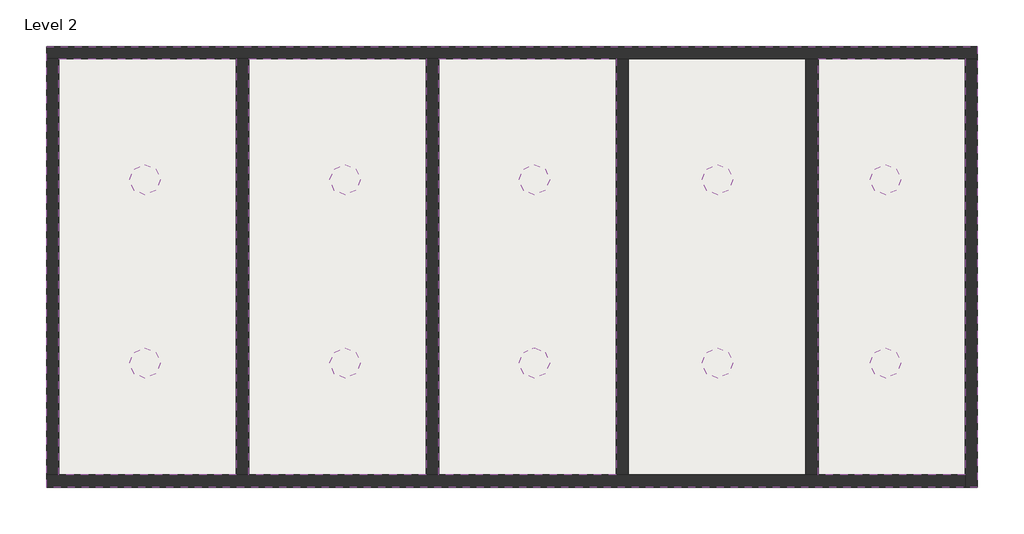
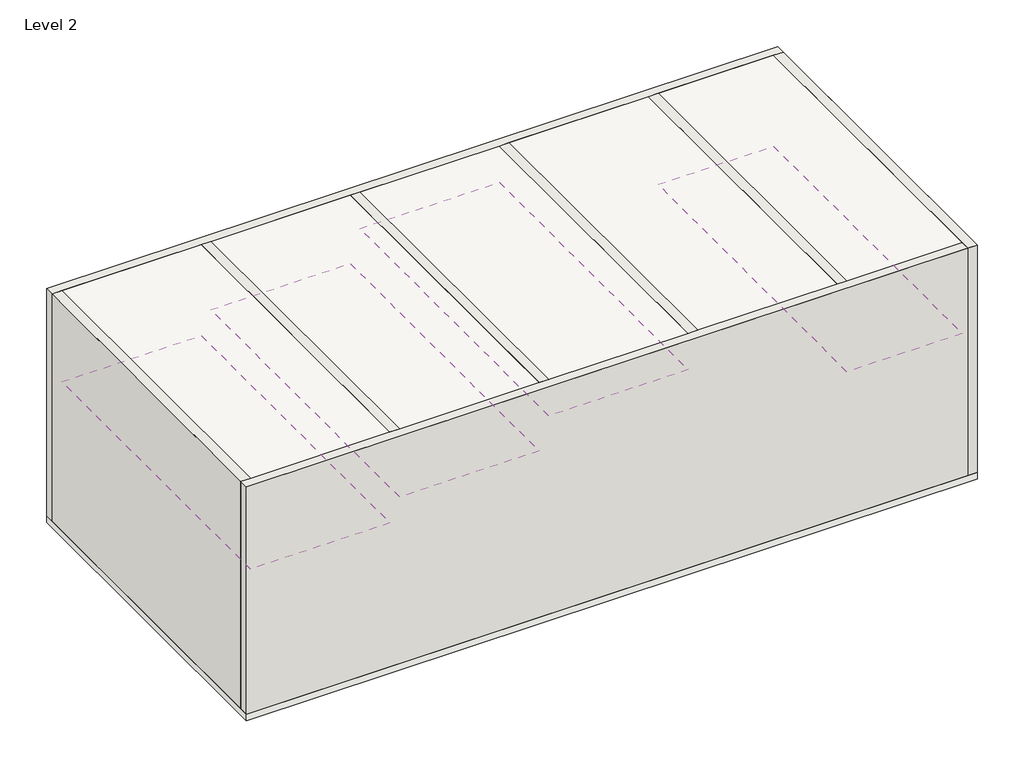
# One storey: 10 light fixtures, 8 walls, 4 coverings, 2 slabs.
"""IFC4 building model written with IfcOpenShell, lengths in millimetres."""

import ifcopenshell
import ifcopenshell.guid

model = None  # the IFC model being written
_history = None  # IfcOwnerHistory: only IFC2X3 demands one
_inside = {}  # id of a spatial element -> (the spatial element, [elements in it])
_under = {}  # id of a project, library or spatial element -> (it, [spatial elements below it])
_declared = {}  # id of a project -> (the project, [libraries it declares])
_typed = {}  # id of a type object -> (the type object, [elements of that type])
_made_of = {}  # id of a material, layer set ... -> (it, [elements and type objects made of it])


def new_model(schema):
    """Start an empty IFC model of exactly this schema.

    Asked for "IFC4X3", IfcOpenShell would pick the latest addendum, in which some entities
    have other attributes; the version numbers below select the first issue.
    IFC2X3 requires an IfcOwnerHistory on every rooted entity: one is made here for all.
    """
    global model, _history
    if schema == "IFC4X3":
        model = ifcopenshell.file(schema_version=(4, 3, 0, 0))
    else:
        model = ifcopenshell.file(schema=schema)
    _inside.clear()
    _under.clear()
    _declared.clear()
    _typed.clear()
    _made_of.clear()
    _history = None
    if model.schema == "IFC2X3":
        org = make("IfcOrganization", Name="unknown")
        user = make(
            "IfcPersonAndOrganization",
            ThePerson=make("IfcPerson", FamilyName="unknown"),
            TheOrganization=org,
        )
        app = make(
            "IfcApplication",
            ApplicationDeveloper=org,
            Version="unknown",
            ApplicationFullName="unknown",
            ApplicationIdentifier="unknown",
        )
        _history = make(
            "IfcOwnerHistory",
            OwningUser=user,
            OwningApplication=app,
            ChangeAction="ADDED",
            CreationDate=0,
        )
    return model


def make(cls, **values):
    """One entity of the class cls with the attributes given. An attribute that is None is left unset."""
    return model.create_entity(
        cls, **{name: value for name, value in values.items() if value is not None}
    )


def rooted(cls, **values):
    """An entity with a GlobalId (a new one), such as an element, a storey or a relation."""
    return make(cls, GlobalId=ifcopenshell.guid.new(), OwnerHistory=_history, **values)


def si_unit(unit_type, name, prefix=None):
    """IfcSIUnit, for example si_unit("LENGTHUNIT", "METRE", prefix="MILLI")."""
    return make("IfcSIUnit", UnitType=unit_type, Prefix=prefix, Name=name)


def assignment(units):
    """IfcUnitAssignment: the units of a project."""
    return None if units is None else make("IfcUnitAssignment", Units=units)


def point(xyz):
    """IfcCartesianPoint."""
    return None if xyz is None else make("IfcCartesianPoint", Coordinates=xyz)


def direction(xyz):
    """IfcDirection."""
    return None if xyz is None else make("IfcDirection", DirectionRatios=xyz)


def frame(location, z_axis=None, x_axis=None):
    """IfcAxis2Placement3D, a coordinate frame: its origin and axes. An axis left out is left unset."""
    return make(
        "IfcAxis2Placement3D",
        Location=point(location),
        Axis=direction(z_axis),
        RefDirection=direction(x_axis),
    )


def frame_2d(location, x_axis=None):
    """IfcAxis2Placement2D, a coordinate frame in the plane: its origin and x axis."""
    return make(
        "IfcAxis2Placement2D", Location=point(location), RefDirection=direction(x_axis)
    )


def origin():
    """The frame at (0, 0, 0) with its axes left unset."""
    return frame((0.0, 0.0, 0.0))


def origin_2d():
    """The frame at (0, 0) in the plane with its x axis left unset."""
    return frame_2d((0.0, 0.0))


def place(relative_to, where):
    """IfcLocalPlacement: puts the frame where relative to a parent placement (None: the world)."""
    return make(
        "IfcLocalPlacement", PlacementRelTo=relative_to, RelativePlacement=where
    )


def context(
    kind, dimensions, precision=None, world=None, true_north=None, identifier=None
):
    """IfcGeometricRepresentationContext, for example the 3D "Model" context."""
    return make(
        "IfcGeometricRepresentationContext",
        ContextIdentifier=identifier,
        ContextType=kind,
        CoordinateSpaceDimension=dimensions,
        Precision=precision,
        WorldCoordinateSystem=world,
        TrueNorth=true_north,
    )


def project(units=None, contexts=None):
    """IfcProject with its units and contexts."""
    return rooted(
        "IfcProject",
        Name="project",
        RepresentationContexts=contexts,
        UnitsInContext=assignment(units),
    )


def spatial(cls, under=None, at=None, **own):
    """A site, building, storey or space (cls), placed at a placement, below another one or the project."""
    s = rooted(cls, ObjectPlacement=at, **own)
    if under is not None:
        _under.setdefault(under.id(), (under, []))[1].append(s)
    return s


def polyline(points):
    """IfcPolyline through the points."""
    return make("IfcPolyline", Points=[point(p) for p in points])


def circle_curve(where, radius):
    """IfcCircle in the frame where."""
    return make("IfcCircle", Position=where, Radius=radius)


def ellipse_curve(where, semi_axis1, semi_axis2):
    """IfcEllipse in the frame where."""
    return make(
        "IfcEllipse", Position=where, SemiAxis1=semi_axis1, SemiAxis2=semi_axis2
    )


def trimmed(basis, trim1, trim2, sense, master):
    """IfcTrimmedCurve: the piece of a basis curve between two trims."""
    return make(
        "IfcTrimmedCurve",
        BasisCurve=basis,
        Trim1=trim1,
        Trim2=trim2,
        SenseAgreement=sense,
        MasterRepresentation=master,
    )


def segment(curve, same_sense, transition):
    """IfcCompositeCurveSegment."""
    return make(
        "IfcCompositeCurveSegment",
        Transition=transition,
        SameSense=same_sense,
        ParentCurve=curve,
    )


def composite_curve(segments, self_intersect=None):
    """IfcCompositeCurve: segments joined end to end."""
    return make("IfcCompositeCurve", Segments=segments, SelfIntersect=self_intersect)


def outline(outer, holes=None, kind="AREA"):
    """IfcArbitraryClosedProfileDef: a profile drawn as a closed curve; with holes, ...WithVoids."""
    if holes is None:
        return make("IfcArbitraryClosedProfileDef", ProfileType=kind, OuterCurve=outer)
    return make(
        "IfcArbitraryProfileDefWithVoids",
        ProfileType=kind,
        OuterCurve=outer,
        InnerCurves=holes,
    )


def extrude(swept, where, along, depth):
    """IfcExtrudedAreaSolid: the profile swept, set in the frame where, extruded along a direction by depth."""
    return make(
        "IfcExtrudedAreaSolid",
        SweptArea=swept,
        Position=where,
        ExtrudedDirection=direction(along),
        Depth=depth,
    )


def faces_of(points, faces, orient=None, outer=None):
    """IfcFace entities. A face is a list of loops; a loop is a list of indices into points, from 0.

    orient and outer hold one flag for each loop. By default every Orientation is true, the
    first loop of a face is its IfcFaceOuterBound and the others are IfcFaceBound.
    """
    made = []
    for i, loops in enumerate(faces):
        bounds = []
        for j, loop in enumerate(loops):
            is_outer = j == 0 if outer is None else outer[i][j]
            bounds.append(
                make(
                    "IfcFaceOuterBound" if is_outer else "IfcFaceBound",
                    Bound=make("IfcPolyLoop", Polygon=[points[k] for k in loop]),
                    Orientation=True if orient is None else orient[i][j],
                )
            )
        made.append(make("IfcFace", Bounds=bounds))
    return made


def faceted_brep(points, faces, orient=None, outer=None, voids=None):
    """IfcFacetedBrep: a solid bounded by flat faces; with voids (closed shells), ...WithVoids."""
    shared = [point(p) for p in points]
    hull = make("IfcClosedShell", CfsFaces=faces_of(shared, faces, orient, outer))
    if voids is None:
        return make("IfcFacetedBrep", Outer=hull)
    return make(
        "IfcFacetedBrepWithVoids",
        Outer=hull,
        Voids=[
            make(cls, CfsFaces=faces_of(shared, fs, o, b)) for cls, fs, o, b in voids
        ],
    )


def shape(context_of_items, identifier, shape_type, items):
    """IfcShapeRepresentation: the items that make up one representation, for example the "Body"."""
    return make(
        "IfcShapeRepresentation",
        ContextOfItems=context_of_items,
        RepresentationIdentifier=identifier,
        RepresentationType=shape_type,
        Items=items,
    )


def source(mapping_origin, context_of_items, identifier, shape_type, items):
    """IfcRepresentationMap: a shape defined once, which mapped items show again and again."""
    return make(
        "IfcRepresentationMap",
        MappingOrigin=mapping_origin,
        MappedRepresentation=shape(context_of_items, identifier, shape_type, items),
    )


def transform(
    local_origin,
    x_axis=None,
    y_axis=None,
    z_axis=None,
    scale=None,
    scale2=None,
    scale3=None,
    uniform=True,
):
    """IfcCartesianTransformationOperator3D, or its non-uniform kind. x_axis, y_axis, z_axis: its Axis1, 2, 3."""
    if uniform:
        return make(
            "IfcCartesianTransformationOperator3D",
            Axis1=direction(x_axis),
            Axis2=direction(y_axis),
            LocalOrigin=point(local_origin),
            Scale=scale,
            Axis3=direction(z_axis),
        )
    return make(
        "IfcCartesianTransformationOperator3DnonUniform",
        Axis1=direction(x_axis),
        Axis2=direction(y_axis),
        LocalOrigin=point(local_origin),
        Scale=scale,
        Axis3=direction(z_axis),
        Scale2=scale2,
        Scale3=scale3,
    )


def mapped(mapping_source, mapping_target):
    """IfcMappedItem: shows the shape of a source again, moved by a transform."""
    return make(
        "IfcMappedItem", MappingSource=mapping_source, MappingTarget=mapping_target
    )


def made_of(thing, what):
    """Note that an element or type object is made of a material, layer set ...; save() writes the relation."""
    if what is not None:
        _made_of.setdefault(what.id(), (what, []))[1].append(thing)
    return thing


def element(
    cls,
    number,
    at=None,
    inside=None,
    cuts=None,
    type_object=None,
    material=None,
    context=None,
    identifier="Body",
    shape_type=None,
    held_by="IfcProductDefinitionShape",
    body=None,
    shapes=None,
    **own,
):
    """One element of the class cls, such as IfcWall. Its Tag is "e" and its number.

    at: its placement. inside: the storey or other place that contains it. cuts: it is an
    opening in that element (IfcRelVoidsElement). A single representation is given by context,
    identifier, shape_type and body (its items); several are given by shapes. held_by: the class
    of the entity that holds the representations. save() writes the other relations.
    """
    e = rooted(cls, Tag="e%d" % number, ObjectPlacement=at, **own)
    if body is not None:
        shapes = [shape(context, identifier, shape_type, body)]
    if shapes is not None:
        e.Representation = make(held_by, Representations=shapes)
    if inside is not None:
        _inside.setdefault(inside.id(), (inside, []))[1].append(e)
    if cuts is not None:
        rooted(
            "IfcRelVoidsElement", RelatingBuildingElement=cuts, RelatedOpeningElement=e
        )
    if type_object is not None:
        _typed.setdefault(type_object.id(), (type_object, []))[1].append(e)
    return made_of(e, material)


def aggregate(whole, parts):
    """IfcRelAggregates: a whole, such as a stair, and the parts it consists of."""
    return rooted("IfcRelAggregates", RelatingObject=whole, RelatedObjects=parts)


def save(model, path):
    """Write the relations noted so far, then the file.

    IfcRelAggregates (storeys below a building ...), IfcRelContainedInSpatialStructure (elements
    in a storey), IfcRelDefinesByType, IfcRelAssociatesMaterial and IfcRelDeclares: one each for
    every whole, place, type object, material and project.
    """
    for whole, parts in _under.values():
        aggregate(whole, parts)
    for where, things in _inside.values():
        rooted(
            "IfcRelContainedInSpatialStructure",
            RelatedElements=things,
            RelatingStructure=where,
        )
    for kind, things in _typed.values():
        rooted("IfcRelDefinesByType", RelatedObjects=things, RelatingType=kind)
    for what, things in _made_of.values():
        rooted("IfcRelAssociatesMaterial", RelatedObjects=things, RelatingMaterial=what)
    for by, libraries in _declared.values():
        rooted("IfcRelDeclares", RelatingContext=by, RelatedDefinitions=libraries)
    model.write(path)


def plane_surface(at):
    """IfcPlane: the flat surface through the origin of the frame at, square to its z axis."""
    return make("IfcPlane", Position=at)


def revolved_surface(curve, axis_point, axis_direction):
    """IfcSurfaceOfRevolution: the curve turned about the line through axis_point along axis_direction."""
    return make(
        "IfcSurfaceOfRevolution",
        SweptCurve=make("IfcArbitraryOpenProfileDef", ProfileType="CURVE", Curve=curve),
        AxisPosition=make("IfcAxis1Placement", Location=point(axis_point), Axis=direction(axis_direction)),
    )


def advanced_brep(points, edges, surfaces, faces):
    """IfcAdvancedBrep: a solid bounded by faces that lie on surfaces and meet in shared edges.

    An edge is (start, end): straight between two places in points (the first is 0);
    or (start, end, curve); or (start, end, curve, False) where it runs against its curve.
    A face is (place in surfaces, loops), or (place, loops, False) where it looks against
    its surface's normal. A loop lists edges by number (the first is 1), with a minus sign
    where the edge is run from its end to its start. The first loop is the outer one.
    """
    corners = [point(p) for p in points]
    vertices = [make("IfcVertexPoint", VertexGeometry=c) for c in corners]
    made = []
    for start, end, *more in edges:
        made.append(
            make(
                "IfcEdgeCurve",
                EdgeStart=vertices[start],
                EdgeEnd=vertices[end],
                EdgeGeometry=more[0] if more else make("IfcPolyline", Points=[corners[start], corners[end]]),
                SameSense=more[1] if len(more) > 1 else True,
            )
        )
    hull = []
    for where, loops, *sense in faces:
        bounds = []
        for j, loop in enumerate(loops):
            ring = [make("IfcOrientedEdge", EdgeElement=made[abs(k) - 1], Orientation=k > 0) for k in loop]
            bounds.append(
                make(
                    "IfcFaceOuterBound" if j == 0 else "IfcFaceBound",
                    Bound=make("IfcEdgeLoop", EdgeList=ring),
                    Orientation=True,
                )
            )
        hull.append(make("IfcAdvancedFace", Bounds=bounds, FaceSurface=surfaces[where], SameSense=sense[0] if sense else True))
    return make("IfcAdvancedBrep", Outer=make("IfcClosedShell", CfsFaces=hull))


def downlight_downlight_e6a68a7d(model_context):
    return source(origin(), model_context, "Body", "SolidModel", [
        advanced_brep(
        [(-230.0, 0.0, 0.0), (230.0, 0.0, 0.0), (0.0, 0.0, 0.0), (0.0, 0.0, 70.3180567)],
        [
            (0, 1, circle_curve(frame((0.0, 0.0, 0.0), z_axis=(0.0, 0.0, -1.0), x_axis=(1.0, 0.0, 0.0)), 230.0)),
            (1, 2),
            (2, 0),
            (1, 0, circle_curve(frame((0.0, 0.0, 0.0), z_axis=(0.0, 0.0, -1.0), x_axis=(1.0, 0.0, 0.0)), 230.0)),
            (3, 1, circle_curve(frame((13.1969865, 0.0, -297.8236248), z_axis=(0.0, 1.0, 0.0), x_axis=(1.0, 0.0, 0.0)), 368.3781456)),
            (0, 3, circle_curve(frame((-13.1969865, 0.0, -297.8236248), z_axis=(0.0, 1.0, 0.0), x_axis=(-1.0, 0.0, 0.0)), 368.3781456)),
        ],
        [
            plane_surface(frame((0.0, 0.0, 0.0), z_axis=(0.0, 0.0, -1.0), x_axis=(1.0, 0.0, 0.0))),
            revolved_surface(trimmed(ellipse_curve(frame((13.1969865, 0.0, -297.8236248), z_axis=(0.0, -1.0, 0.0), x_axis=(1.0, 0.0, 0.0)), 368.3781456, 368.3781456), [point((230.0, 0.0, 0.0))], [point((0.0, 0.0, 70.3180567))], True, "CARTESIAN"), (0.0, 0.0, 2194.0651339), (0.0, 0.0, 1.0)),
        ],
        [
            (0, [[1, 2, 3]]),
            (0, [[4, -3, -2]]),
            (1, [[5, -1, 6]]),
            (1, [[-6, -4, -5]]),
        ],
    ),
        extrude(outline(composite_curve([segment(trimmed(circle_curve(origin_2d(), 250.0), [point((-250.0, 0.0))], [point((250.0, 0.0))], False, "CARTESIAN"), True, "CONTINUOUS"), segment(trimmed(circle_curve(origin_2d(), 250.0), [point((250.0, 0.0))], [point((-250.0, 0.0))], False, "CARTESIAN"), True, "CONTINUOUS")], self_intersect=False)), frame((0.0, 0.0, -10.1537533), z_axis=(0.0, 0.0, 1.0), x_axis=(1.0, 0.0, 0.0)), (0.0, 0.0, 1.0), 10.1537533),
    ])


model = new_model("IFC4")

# Units and contexts
model_context = context("Model", 3, world=origin())
ifc_project = project(units=[si_unit("LENGTHUNIT", "METRE", prefix="MILLI")], contexts=[model_context])

# Site, building, storey
site = spatial("IfcSite", under=ifc_project)
building = spatial("IfcBuilding", under=site)
storey = spatial("IfcBuildingStorey", under=building, Name="Level 2", Elevation=5000.0)

# Coverings
placement = place(None, origin())
element("IfcCovering", 1, ObjectType="Plain", at=placement, inside=storey, context=model_context, shape_type="SweptSolid", body=[
    extrude(outline(polyline([(4711.6370984, -2494.7382368), (4711.6370984, 4305.2617632), (7111.6370984, 4305.2617632), (7111.6370984, -2494.7382368), (4711.6370984, -2494.7382368)])), frame((0.0, 0.0, 8000.0), z_axis=(0.0, 0.0, 1.0), x_axis=(1.0, 0.0, 0.0)), (0.0, 0.0, 1.0), 57.0),
])
element("IfcCovering", 2, ObjectType="Plain", at=placement, inside=storey, context=model_context, shape_type="SweptSolid", body=[
    extrude(outline(polyline([(-1488.3629016, -2494.7382368), (-1488.3629016, 4305.2617632), (1411.6370984, 4305.2617632), (1411.6370984, -2494.7382368), (-1488.3629016, -2494.7382368)])), frame((0.0, 0.0, 9200.0), z_axis=(0.0, 0.0, 1.0), x_axis=(1.0, 0.0, 0.0)), (0.0, 0.0, 1.0), 57.0),
])
element("IfcCovering", 3, ObjectType="Plain", at=placement, inside=storey, context=model_context, shape_type="SweptSolid", body=[
    extrude(outline(polyline([(-4588.3629016, -2494.7382368), (-4588.3629016, 4305.2617632), (-1688.3629016, 4305.2617632), (-1688.3629016, -2494.7382368), (-4588.3629016, -2494.7382368)])), frame((0.0, 0.0, 8500.0), z_axis=(0.0, 0.0, 1.0), x_axis=(1.0, 0.0, 0.0)), (0.0, 0.0, 1.0), 57.0),
])
element("IfcCovering", 4, ObjectType="Plain", at=placement, inside=storey, context=model_context, shape_type="SweptSolid", body=[
    extrude(outline(polyline([(-7688.3629016, 4305.2617632), (-4788.3629016, 4305.2617632), (-4788.3629016, -2494.7382368), (-7688.3629016, -2494.7382368), (-7688.3629016, 4305.2617632)])), frame((0.0, 0.0, 8000.0), z_axis=(0.0, 0.0, 1.0), x_axis=(1.0, 0.0, 0.0)), (0.0, 0.0, 1.0), 57.0),
])

# Light fixtures
downlight_downlight_shape = downlight_downlight_e6a68a7d(model_context)
element("IfcLightFixture", 5, ObjectType="Downlight : Downlight", at=placement, inside=storey, context=model_context, shape_type="MappedRepresentation", body=[
    mapped(downlight_downlight_shape, transform((-6281.2033206, -666.9973068, 7700.0), x_axis=(1.0, 0.0, 0.0), y_axis=(0.0, 1.0, 0.0), z_axis=(0.0, 0.0, 1.0))),
])
element("IfcLightFixture", 6, ObjectType="Downlight : Downlight", at=placement, inside=storey, context=model_context, shape_type="MappedRepresentation", body=[
    mapped(downlight_downlight_shape, transform((-6281.2033206, 2328.2026932, 7700.0), x_axis=(1.0, 0.0, 0.0), y_axis=(0.0, 1.0, 0.0), z_axis=(0.0, 0.0, 1.0))),
])
element("IfcLightFixture", 7, ObjectType="Downlight : Downlight", at=placement, inside=storey, context=model_context, shape_type="MappedRepresentation", body=[
    mapped(downlight_downlight_shape, transform((-3013.7777439, -666.9973068, 8800.0), x_axis=(1.0, 0.0, 0.0), y_axis=(0.0, 1.0, 0.0), z_axis=(0.0, 0.0, 1.0))),
])
element("IfcLightFixture", 8, ObjectType="Downlight : Downlight", at=placement, inside=storey, context=model_context, shape_type="MappedRepresentation", body=[
    mapped(downlight_downlight_shape, transform((-3013.7777439, 2328.2026932, 8800.0), x_axis=(1.0, 0.0, 0.0), y_axis=(0.0, 1.0, 0.0), z_axis=(0.0, 0.0, 1.0))),
])
element("IfcLightFixture", 9, ObjectType="Downlight : Downlight", at=placement, inside=storey, context=model_context, shape_type="MappedRepresentation", body=[
    mapped(downlight_downlight_shape, transform((76.5388311, -666.9973068, 8500.0), x_axis=(1.0, 0.0, 0.0), y_axis=(0.0, 1.0, 0.0), z_axis=(0.0, 0.0, 1.0))),
])
element("IfcLightFixture", 10, ObjectType="Downlight : Downlight", at=placement, inside=storey, context=model_context, shape_type="MappedRepresentation", body=[
    mapped(downlight_downlight_shape, transform((76.5388311, 2328.2026932, 8500.0), x_axis=(1.0, 0.0, 0.0), y_axis=(0.0, 1.0, 0.0), z_axis=(0.0, 0.0, 1.0))),
])
element("IfcLightFixture", 11, ObjectType="Downlight : Downlight", at=placement, inside=storey, context=model_context, shape_type="MappedRepresentation", body=[
    mapped(downlight_downlight_shape, transform((3067.3545284, -666.9973068, 8900.0), x_axis=(1.0, 0.0, 0.0), y_axis=(0.0, 1.0, 0.0), z_axis=(0.0, 0.0, 1.0))),
])
element("IfcLightFixture", 12, ObjectType="Downlight : Downlight", at=placement, inside=storey, context=model_context, shape_type="MappedRepresentation", body=[
    mapped(downlight_downlight_shape, transform((3067.3545284, 2328.2026932, 8900.0), x_axis=(1.0, 0.0, 0.0), y_axis=(0.0, 1.0, 0.0), z_axis=(0.0, 0.0, 1.0))),
])
element("IfcLightFixture", 13, ObjectType="Downlight : Downlight", at=placement, inside=storey, context=model_context, shape_type="MappedRepresentation", body=[
    mapped(downlight_downlight_shape, transform((5810.7393139, -666.9973068, 8000.0), x_axis=(1.0, 0.0, 0.0), y_axis=(0.0, 1.0, 0.0), z_axis=(0.0, 0.0, 1.0))),
])
element("IfcLightFixture", 14, ObjectType="Downlight : Downlight", at=placement, inside=storey, context=model_context, shape_type="MappedRepresentation", body=[
    mapped(downlight_downlight_shape, transform((5810.7393139, 2328.2026932, 8000.0), x_axis=(1.0, 0.0, 0.0), y_axis=(0.0, 1.0, 0.0), z_axis=(0.0, 0.0, 1.0))),
])

# Slabs
element("IfcSlab", 15, ObjectType="Generic 150mm", at=placement, inside=storey, context=model_context, shape_type="SweptSolid", body=[
    extrude(outline(polyline([(7311.6370984, 4505.2617632), (7311.6370984, -2694.7382368), (-7888.3629016, -2694.7382368), (-7888.3629016, 4505.2617632), (7311.6370984, 4505.2617632)])), frame((0.0, 0.0, 4850.0), z_axis=(0.0, 0.0, 1.0), x_axis=(1.0, 0.0, 0.0)), (0.0, 0.0, 1.0), 150.0),
])
element("IfcSlab", 16, ObjectType="Generic 150mm", at=placement, inside=storey, context=model_context, shape_type="SweptSolid", body=[
    extrude(outline(polyline([(7311.6370984, 4505.2617632), (7311.6370984, -2694.7382368), (-7888.3629016, -2694.7382368), (-7888.3629016, 4505.2617632), (7311.6370984, 4505.2617632)])), frame((0.0, 0.0, 9850.0), z_axis=(0.0, 0.0, 1.0), x_axis=(1.0, 0.0, 0.0)), (0.0, 0.0, 1.0), 150.0),
])

# Walls
element("IfcWall", 17, ObjectType="Generic - 200mm", at=placement, inside=storey, context=model_context, shape_type="Brep", body=[
    faceted_brep([(-7888.3629016, 4305.2617632, 5000.0), (-7688.3629016, 4305.2617632, 5000.0), (-4788.3629016, 4305.2617632, 5000.0), (-4588.3629016, 4305.2617632, 5000.0), (-1688.3629016, 4305.2617632, 5000.0), (-1488.3629016, 4305.2617632, 5000.0), (1411.6370984, 4305.2617632, 5000.0), (1611.6370984, 4305.2617632, 5000.0), (4511.6370984, 4305.2617632, 5000.0), (4711.6370984, 4305.2617632, 5000.0), (7111.6370984, 4305.2617632, 5000.0), (7311.6370984, 4305.2617632, 5000.0), (7311.6370984, 4305.2617632, 10000.0), (7111.6370984, 4305.2617632, 10000.0), (4711.6370984, 4305.2617632, 10000.0), (4511.6370984, 4305.2617632, 10000.0), (1611.6370984, 4305.2617632, 10000.0), (1411.6370984, 4305.2617632, 10000.0), (-1488.3629016, 4305.2617632, 10000.0), (-1688.3629016, 4305.2617632, 10000.0), (-4588.3629016, 4305.2617632, 10000.0), (-4788.3629016, 4305.2617632, 10000.0), (-7688.3629016, 4305.2617632, 10000.0), (-7888.3629016, 4305.2617632, 10000.0), (-7888.3629016, 4505.2617632, 5000.0), (-7888.3629016, 4505.2617632, 10000.0), (7311.6370984, 4505.2617632, 10000.0), (7311.6370984, 4505.2617632, 5000.0)], [[[0, 1, 2, 3, 4, 5, 6, 7, 8, 9, 10, 11, 12, 13, 14, 15, 16, 17, 18, 19, 20, 21, 22, 23]], [[24, 25, 26, 27]], [[11, 10, 9, 8, 7, 6, 5, 4, 3, 2, 1, 0, 24, 27]], [[23, 22, 21, 20, 19, 18, 17, 16, 15, 14, 13, 12, 26, 25]], [[12, 11, 27, 26]], [[0, 23, 25, 24]]]),
])
element("IfcWall", 18, ObjectType="Generic - 200mm", at=placement, inside=storey, context=model_context, shape_type="Brep", body=[
    faceted_brep([(7111.6370984, 4305.2617632, 5000.0), (7111.6370984, -2494.7382368, 5000.0), (7111.6370984, -2694.7382368, 5000.0), (7111.6370984, -2694.7382368, 10000.0), (7111.6370984, -2494.7382368, 10000.0), (7111.6370984, 4305.2617632, 10000.0), (7311.6370984, 4305.2617632, 5000.0), (7311.6370984, 4305.2617632, 10000.0), (7311.6370984, -2694.7382368, 10000.0), (7311.6370984, -2694.7382368, 5000.0)], [[[0, 1, 2, 3, 4, 5]], [[6, 7, 8, 9]], [[2, 1, 0, 6, 9]], [[5, 4, 3, 8, 7]], [[0, 5, 7, 6]], [[3, 2, 9, 8]]]),
])
element("IfcWall", 19, ObjectType="Generic - 200mm", at=placement, inside=storey, context=model_context, shape_type="Brep", body=[
    faceted_brep([(7111.6370984, -2494.7382368, 5000.0), (4711.6370984, -2494.7382368, 5000.0), (4511.6370984, -2494.7382368, 5000.0), (1611.6370984, -2494.7382368, 5000.0), (1411.6370984, -2494.7382368, 5000.0), (-1488.3629016, -2494.7382368, 5000.0), (-1688.3629016, -2494.7382368, 5000.0), (-4588.3629016, -2494.7382368, 5000.0), (-4788.3629016, -2494.7382368, 5000.0), (-7688.3629016, -2494.7382368, 5000.0), (-7888.3629016, -2494.7382368, 5000.0), (-7888.3629016, -2494.7382368, 10000.0), (-7688.3629016, -2494.7382368, 10000.0), (-4788.3629016, -2494.7382368, 10000.0), (-4588.3629016, -2494.7382368, 10000.0), (-1688.3629016, -2494.7382368, 10000.0), (-1488.3629016, -2494.7382368, 10000.0), (1411.6370984, -2494.7382368, 10000.0), (1611.6370984, -2494.7382368, 10000.0), (4511.6370984, -2494.7382368, 10000.0), (4711.6370984, -2494.7382368, 10000.0), (7111.6370984, -2494.7382368, 10000.0), (7111.6370984, -2694.7382368, 5000.0), (7111.6370984, -2694.7382368, 10000.0), (-7888.3629016, -2694.7382368, 10000.0), (-7888.3629016, -2694.7382368, 5000.0)], [[[0, 1, 2, 3, 4, 5, 6, 7, 8, 9, 10, 11, 12, 13, 14, 15, 16, 17, 18, 19, 20, 21]], [[22, 23, 24, 25]], [[10, 9, 8, 7, 6, 5, 4, 3, 2, 1, 0, 22, 25]], [[21, 20, 19, 18, 17, 16, 15, 14, 13, 12, 11, 24, 23]], [[0, 21, 23, 22]], [[11, 10, 25, 24]]]),
])
element("IfcWall", 20, ObjectType="Generic - 200mm", at=placement, inside=storey, context=model_context, shape_type="SweptSolid", body=[
    extrude(outline(polyline([(-7688.3629016, 4305.2617632), (-7688.3629016, -2494.7382368), (-7888.3629016, -2494.7382368), (-7888.3629016, 4305.2617632), (-7688.3629016, 4305.2617632)])), frame((0.0, 0.0, 5000.0), z_axis=(0.0, 0.0, 1.0), x_axis=(1.0, 0.0, 0.0)), (0.0, 0.0, 1.0), 5000.0),
])
element("IfcWall", 21, ObjectType="Generic - 200mm", at=placement, inside=storey, context=model_context, shape_type="SweptSolid", body=[
    extrude(outline(polyline([(-4788.3629016, -2494.7382368), (-4788.3629016, 4305.2617632), (-4588.3629016, 4305.2617632), (-4588.3629016, -2494.7382368), (-4788.3629016, -2494.7382368)])), frame((0.0, 0.0, 5000.0), z_axis=(0.0, 0.0, 1.0), x_axis=(1.0, 0.0, 0.0)), (0.0, 0.0, 1.0), 5000.0),
])
element("IfcWall", 22, ObjectType="Generic - 200mm", at=placement, inside=storey, context=model_context, shape_type="SweptSolid", body=[
    extrude(outline(polyline([(-1688.3629016, -2494.7382368), (-1688.3629016, 4305.2617632), (-1488.3629016, 4305.2617632), (-1488.3629016, -2494.7382368), (-1688.3629016, -2494.7382368)])), frame((0.0, 0.0, 5000.0), z_axis=(0.0, 0.0, 1.0), x_axis=(1.0, 0.0, 0.0)), (0.0, 0.0, 1.0), 5000.0),
])
element("IfcWall", 23, ObjectType="Generic - 200mm", at=placement, inside=storey, context=model_context, shape_type="SweptSolid", body=[
    extrude(outline(polyline([(1411.6370984, -2494.7382368), (1411.6370984, 4305.2617632), (1611.6370984, 4305.2617632), (1611.6370984, -2494.7382368), (1411.6370984, -2494.7382368)])), frame((0.0, 0.0, 5000.0), z_axis=(0.0, 0.0, 1.0), x_axis=(1.0, 0.0, 0.0)), (0.0, 0.0, 1.0), 5000.0),
])
element("IfcWall", 24, ObjectType="Generic - 200mm", at=placement, inside=storey, context=model_context, shape_type="SweptSolid", body=[
    extrude(outline(polyline([(4511.6370984, -2494.7382368), (4511.6370984, 4305.2617632), (4711.6370984, 4305.2617632), (4711.6370984, -2494.7382368), (4511.6370984, -2494.7382368)])), frame((0.0, 0.0, 5000.0), z_axis=(0.0, 0.0, 1.0), x_axis=(1.0, 0.0, 0.0)), (0.0, 0.0, 1.0), 5000.0),
])

save(model, "model.ifc")

# Revit data of these elements
# Type "Plain"
#   built-in parameter 1002203 = 1 (stored number, unit not read)
#   built-in parameter 1002202 = 1 (stored number, unit not read)
#   Layers, outside or top first: 0.045 m "Metal Stud Layer" (function 1); 0.012 m "Gypsum Wall Board" (function 1)
# Type "Downlight : Downlight"
#   Default Elevation = 0
# Type "Generic 150mm"
#   Function = 0
#   Layers, outside or top first: 0.15 m no material (function 1)
# Type "Generic - 200mm"
#   Layers, outside or top first: 0.2 m no material (function 1)
# Elements 1, 4 (IfcCovering, "Plain")
#   Height Offset From Level = 3 m
#   Phase Created = New Construction
#   Materials on its faces: "Gypsum Wall Board", "Metal Stud Layer"
# Element 2 (IfcCovering, "Plain")
#   Height Offset From Level = 4.2 m
#   Phase Created = New Construction
#   Materials on its faces: "Gypsum Wall Board", "Metal Stud Layer"
# Element 3 (IfcCovering, "Plain")
#   Height Offset From Level = 3.5 m
#   Phase Created = New Construction
#   Materials on its faces: "Gypsum Wall Board", "Metal Stud Layer"
# Element 5 (IfcLightFixture, "Downlight : Downlight")
#   Mark = "45"
#   Phase Created = New Construction
# Element 6 (IfcLightFixture, "Downlight : Downlight")
#   Mark = "46"
#   Phase Created = New Construction
# Element 7 (IfcLightFixture, "Downlight : Downlight")
#   Mark = "47"
#   Phase Created = New Construction
# Element 8 (IfcLightFixture, "Downlight : Downlight")
#   Mark = "48"
#   Phase Created = New Construction
# Element 9 (IfcLightFixture, "Downlight : Downlight")
#   Mark = "49"
#   Phase Created = New Construction
# Element 10 (IfcLightFixture, "Downlight : Downlight")
#   Mark = "50"
#   Phase Created = New Construction
# Element 11 (IfcLightFixture, "Downlight : Downlight")
#   Mark = "51"
#   Phase Created = New Construction
# Element 12 (IfcLightFixture, "Downlight : Downlight")
#   Mark = "52"
#   Phase Created = New Construction
# Element 13 (IfcLightFixture, "Downlight : Downlight")
#   Mark = "53"
#   Phase Created = New Construction
# Element 14 (IfcLightFixture, "Downlight : Downlight")
#   Mark = "54"
#   Phase Created = New Construction
# Element 15 (IfcSlab, "Generic 150mm")
#   Height Offset From Level = 0 m
#   Phase Created = New Construction
#   Materials on its faces: "Default Floor"
# Element 16 (IfcSlab, "Generic 150mm")
#   Height Offset From Level = 5 m
#   Phase Created = New Construction
#   Materials on its faces: "Default Floor"
# Elements 17, 18, 19, 20, 21, 22, 23, 24 (IfcWall, "Generic - 200mm")
#   Top Offset = 5 m
#   Base Offset = 0 m
#   wall height = 5 m
#   Phase Created = New Construction
#   Base Constraint = Level 2
#   Top Constraint = Level 2
#   Materials on its faces: "Default Wall"
# Materials
#   "Metal Stud Layer": class "Metal", colour RGB 127 127 127, transparency 0, Description = "Light gauge steel framing, thermal air layer", Cost = 0
#   "Gypsum Wall Board": class "Generic", colour RGB 249 249 249, transparency 0, Description = "Gypsum Wall Board", Cost = 0
#   "Default Floor": class "Miscellaneous", colour RGB 127 127 127, transparency 0, Cost = 0
#   "Default Wall": class "Miscellaneous", colour RGB 128 128 128, transparency 0, Cost = 0
